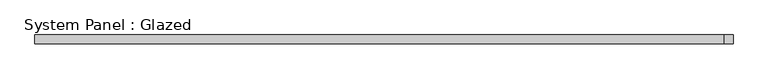
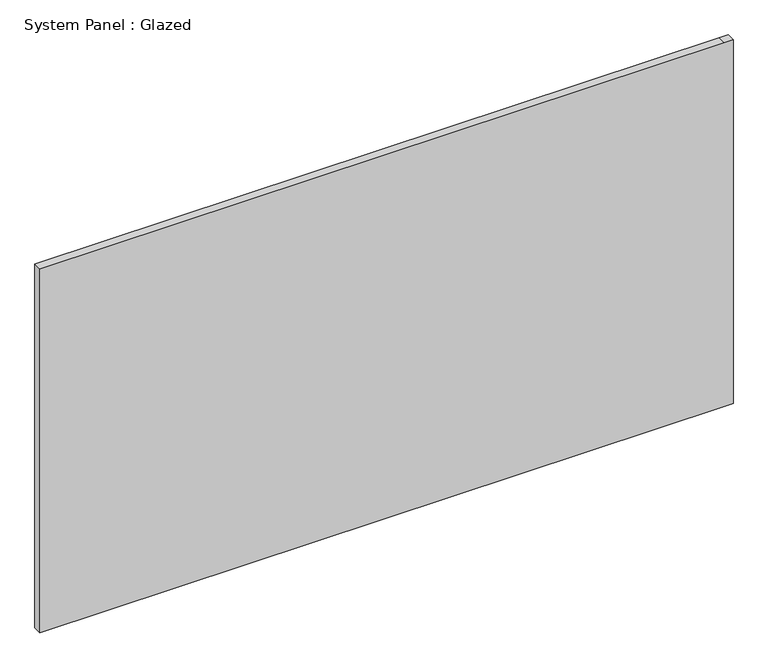
"""IFC4 building model written with IfcOpenShell, lengths in millimetres: plate geometry, System Panel : Glazed."""

import ifcopenshell
import ifcopenshell.guid

model = None  # the IFC model being written
_history = None  # IfcOwnerHistory: only IFC2X3 demands one
_inside = {}  # id of a spatial element -> (the spatial element, [elements in it])
_under = {}  # id of a project, library or spatial element -> (it, [spatial elements below it])
_declared = {}  # id of a project -> (the project, [libraries it declares])
_typed = {}  # id of a type object -> (the type object, [elements of that type])
_made_of = {}  # id of a material, layer set ... -> (it, [elements and type objects made of it])


def new_model(schema):
    """Start an empty IFC model of exactly this schema.

    Asked for "IFC4X3", IfcOpenShell would pick the latest addendum, in which some entities
    have other attributes; the version numbers below select the first issue.
    IFC2X3 requires an IfcOwnerHistory on every rooted entity: one is made here for all.
    """
    global model, _history
    if schema == "IFC4X3":
        model = ifcopenshell.file(schema_version=(4, 3, 0, 0))
    else:
        model = ifcopenshell.file(schema=schema)
    _inside.clear()
    _under.clear()
    _declared.clear()
    _typed.clear()
    _made_of.clear()
    _history = None
    if model.schema == "IFC2X3":
        org = make("IfcOrganization", Name="unknown")
        user = make(
            "IfcPersonAndOrganization",
            ThePerson=make("IfcPerson", FamilyName="unknown"),
            TheOrganization=org,
        )
        app = make(
            "IfcApplication",
            ApplicationDeveloper=org,
            Version="unknown",
            ApplicationFullName="unknown",
            ApplicationIdentifier="unknown",
        )
        _history = make(
            "IfcOwnerHistory",
            OwningUser=user,
            OwningApplication=app,
            ChangeAction="ADDED",
            CreationDate=0,
        )
    return model


def make(cls, **values):
    """One entity of the class cls with the attributes given. An attribute that is None is left unset."""
    return model.create_entity(
        cls, **{name: value for name, value in values.items() if value is not None}
    )


def rooted(cls, **values):
    """An entity with a GlobalId (a new one), such as an element, a storey or a relation."""
    return make(cls, GlobalId=ifcopenshell.guid.new(), OwnerHistory=_history, **values)


def si_unit(unit_type, name, prefix=None):
    """IfcSIUnit, for example si_unit("LENGTHUNIT", "METRE", prefix="MILLI")."""
    return make("IfcSIUnit", UnitType=unit_type, Prefix=prefix, Name=name)


def assignment(units):
    """IfcUnitAssignment: the units of a project."""
    return None if units is None else make("IfcUnitAssignment", Units=units)


def point(xyz):
    """IfcCartesianPoint."""
    return None if xyz is None else make("IfcCartesianPoint", Coordinates=xyz)


def direction(xyz):
    """IfcDirection."""
    return None if xyz is None else make("IfcDirection", DirectionRatios=xyz)


def frame(location, z_axis=None, x_axis=None):
    """IfcAxis2Placement3D, a coordinate frame: its origin and axes. An axis left out is left unset."""
    return make(
        "IfcAxis2Placement3D",
        Location=point(location),
        Axis=direction(z_axis),
        RefDirection=direction(x_axis),
    )


def origin():
    """The frame at (0, 0, 0) with its axes left unset."""
    return frame((0.0, 0.0, 0.0))


def place(relative_to, where):
    """IfcLocalPlacement: puts the frame where relative to a parent placement (None: the world)."""
    return make(
        "IfcLocalPlacement", PlacementRelTo=relative_to, RelativePlacement=where
    )


def context(
    kind, dimensions, precision=None, world=None, true_north=None, identifier=None
):
    """IfcGeometricRepresentationContext, for example the 3D "Model" context."""
    return make(
        "IfcGeometricRepresentationContext",
        ContextIdentifier=identifier,
        ContextType=kind,
        CoordinateSpaceDimension=dimensions,
        Precision=precision,
        WorldCoordinateSystem=world,
        TrueNorth=true_north,
    )


def project(units=None, contexts=None):
    """IfcProject with its units and contexts."""
    return rooted(
        "IfcProject",
        Name="project",
        RepresentationContexts=contexts,
        UnitsInContext=assignment(units),
    )


def spatial(cls, under=None, at=None, **own):
    """A site, building, storey or space (cls), placed at a placement, below another one or the project."""
    s = rooted(cls, ObjectPlacement=at, **own)
    if under is not None:
        _under.setdefault(under.id(), (under, []))[1].append(s)
    return s


def polyline(points):
    """IfcPolyline through the points."""
    return make("IfcPolyline", Points=[point(p) for p in points])


def outline(outer, holes=None, kind="AREA"):
    """IfcArbitraryClosedProfileDef: a profile drawn as a closed curve; with holes, ...WithVoids."""
    if holes is None:
        return make("IfcArbitraryClosedProfileDef", ProfileType=kind, OuterCurve=outer)
    return make(
        "IfcArbitraryProfileDefWithVoids",
        ProfileType=kind,
        OuterCurve=outer,
        InnerCurves=holes,
    )


def extrude(swept, where, along, depth):
    """IfcExtrudedAreaSolid: the profile swept, set in the frame where, extruded along a direction by depth."""
    return make(
        "IfcExtrudedAreaSolid",
        SweptArea=swept,
        Position=where,
        ExtrudedDirection=direction(along),
        Depth=depth,
    )


def shape(context_of_items, identifier, shape_type, items):
    """IfcShapeRepresentation: the items that make up one representation, for example the "Body"."""
    return make(
        "IfcShapeRepresentation",
        ContextOfItems=context_of_items,
        RepresentationIdentifier=identifier,
        RepresentationType=shape_type,
        Items=items,
    )


def source(mapping_origin, context_of_items, identifier, shape_type, items):
    """IfcRepresentationMap: a shape defined once, which mapped items show again and again."""
    return make(
        "IfcRepresentationMap",
        MappingOrigin=mapping_origin,
        MappedRepresentation=shape(context_of_items, identifier, shape_type, items),
    )


def transform(
    local_origin,
    x_axis=None,
    y_axis=None,
    z_axis=None,
    scale=None,
    scale2=None,
    scale3=None,
    uniform=True,
):
    """IfcCartesianTransformationOperator3D, or its non-uniform kind. x_axis, y_axis, z_axis: its Axis1, 2, 3."""
    if uniform:
        return make(
            "IfcCartesianTransformationOperator3D",
            Axis1=direction(x_axis),
            Axis2=direction(y_axis),
            LocalOrigin=point(local_origin),
            Scale=scale,
            Axis3=direction(z_axis),
        )
    return make(
        "IfcCartesianTransformationOperator3DnonUniform",
        Axis1=direction(x_axis),
        Axis2=direction(y_axis),
        LocalOrigin=point(local_origin),
        Scale=scale,
        Axis3=direction(z_axis),
        Scale2=scale2,
        Scale3=scale3,
    )


def mapped(mapping_source, mapping_target):
    """IfcMappedItem: shows the shape of a source again, moved by a transform."""
    return make(
        "IfcMappedItem", MappingSource=mapping_source, MappingTarget=mapping_target
    )


def made_of(thing, what):
    """Note that an element or type object is made of a material, layer set ...; save() writes the relation."""
    if what is not None:
        _made_of.setdefault(what.id(), (what, []))[1].append(thing)
    return thing


def element(
    cls,
    number,
    at=None,
    inside=None,
    cuts=None,
    type_object=None,
    material=None,
    context=None,
    identifier="Body",
    shape_type=None,
    held_by="IfcProductDefinitionShape",
    body=None,
    shapes=None,
    **own,
):
    """One element of the class cls, such as IfcWall. Its Tag is "e" and its number.

    at: its placement. inside: the storey or other place that contains it. cuts: it is an
    opening in that element (IfcRelVoidsElement). A single representation is given by context,
    identifier, shape_type and body (its items); several are given by shapes. held_by: the class
    of the entity that holds the representations. save() writes the other relations.
    """
    e = rooted(cls, Tag="e%d" % number, ObjectPlacement=at, **own)
    if body is not None:
        shapes = [shape(context, identifier, shape_type, body)]
    if shapes is not None:
        e.Representation = make(held_by, Representations=shapes)
    if inside is not None:
        _inside.setdefault(inside.id(), (inside, []))[1].append(e)
    if cuts is not None:
        rooted(
            "IfcRelVoidsElement", RelatingBuildingElement=cuts, RelatedOpeningElement=e
        )
    if type_object is not None:
        _typed.setdefault(type_object.id(), (type_object, []))[1].append(e)
    return made_of(e, material)


def aggregate(whole, parts):
    """IfcRelAggregates: a whole, such as a stair, and the parts it consists of."""
    return rooted("IfcRelAggregates", RelatingObject=whole, RelatedObjects=parts)


def save(model, path):
    """Write the relations noted so far, then the file.

    IfcRelAggregates (storeys below a building ...), IfcRelContainedInSpatialStructure (elements
    in a storey), IfcRelDefinesByType, IfcRelAssociatesMaterial and IfcRelDeclares: one each for
    every whole, place, type object, material and project.
    """
    for whole, parts in _under.values():
        aggregate(whole, parts)
    for where, things in _inside.values():
        rooted(
            "IfcRelContainedInSpatialStructure",
            RelatedElements=things,
            RelatingStructure=where,
        )
    for kind, things in _typed.values():
        rooted("IfcRelDefinesByType", RelatedObjects=things, RelatingType=kind)
    for what, things in _made_of.values():
        rooted("IfcRelAssociatesMaterial", RelatedObjects=things, RelatingMaterial=what)
    for by, libraries in _declared.values():
        rooted("IfcRelDeclares", RelatingContext=by, RelatedDefinitions=libraries)
    model.write(path)


def system_panel_glazed_d6bfc804(model_context):
    return source(origin(), model_context, "Body", "SweptSolid", [
        extrude(outline(polyline([(0.0, -1012.825), (0.0, 987.425), (0.0, 1012.825), (1123.95, 1012.825), (1123.95, 987.425), (1123.95, -1012.825), (0.0, -1012.825)])), frame((0.0, -44.45, 0.0), z_axis=(0.0, 1.0, 0.0), x_axis=(0.0, 0.0, 1.0)), (0.0, 0.0, 1.0), 25.4),
    ])


if __name__ == "__main__":
    model = new_model("IFC4")
    model_context = context("Model", 3, world=origin())
    ifc_project = project(units=[si_unit("LENGTHUNIT", "METRE", prefix="MILLI")], contexts=[model_context])
    site = spatial("IfcSite", under=ifc_project)
    building = spatial("IfcBuilding", under=site)
    placement = place(None, origin())
    system_panel_glazed_shape = system_panel_glazed_d6bfc804(model_context)
    element("IfcPlate", 1, ObjectType="System Panel : Glazed", at=placement, inside=building, context=model_context, shape_type="MappedRepresentation", body=[
        mapped(system_panel_glazed_shape, transform((0.0, 0.0, 0.0), x_axis=(1.0, 0.0, 0.0), y_axis=(0.0, 1.0, 0.0), z_axis=(0.0, 0.0, 1.0))),
    ])
    save(model, "model.ifc")

# Revit data of these elements
# Element 1 (IfcPlate, "System Panel : Glazed")
#   Materials on its faces: "Glass"
# Materials
#   "Glass": class "Glass", colour RGB 0 128 192, transparency 0.75
